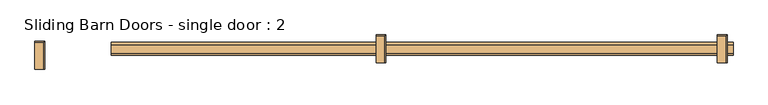
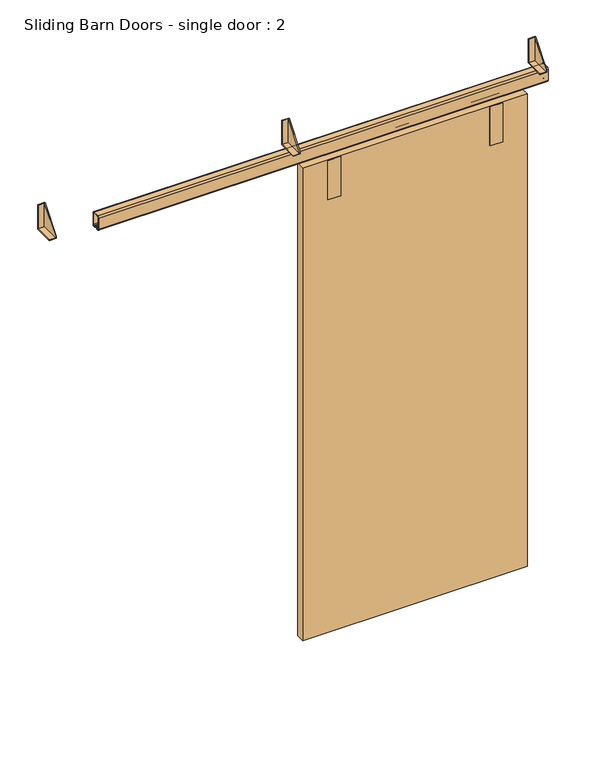
"""IFC4 building model written with IfcOpenShell, lengths in millimetres: door geometry, Sliding Barn Doors - single door : 2."""

from ifc_helpers import new_model, si_unit, point, frame, frame_2d, origin, place, context, project, spatial, polyline, circle_curve, trimmed, segment, composite_curve, outline, extrude, source, transform, mapped, element, save


def sliding_barn_doors_single_door_2_8c843bd4(model_context):
    return source(origin(), model_context, "Body", "SweptSolid", [
        extrude(outline(polyline([(-158.75, 2152.65), (-79.375, 2247.773), (-79.375, 2146.3), (-158.75, 2146.3), (-158.75, 2152.65)])), frame((-1487.5371094, 0.0, 0.0), z_axis=(1.0, 0.0, 0.0), x_axis=(0.0, 1.0, 0.0)), (0.0, 0.0, 1.0), 3.175),
        extrude(outline(polyline([(-76.2, 2143.125), (-158.75, 2143.125), (-158.75, 2146.3), (-79.375, 2146.3), (-79.375, 2247.773), (-76.2, 2247.773), (-76.2, 2143.125)])), frame((-1512.8378906, 0.0, 0.0), z_axis=(1.0, 0.0, 0.0), x_axis=(0.0, 1.0, 0.0)), (0.0, 0.0, 1.0), 28.4757812),
        extrude(outline(polyline([(-139.7, 2152.65), (-60.325, 2247.773), (-60.325, 2146.3), (-139.7, 2146.3), (-139.7, 2152.65)])), frame((-484.2371094, 0.0, 0.0), z_axis=(1.0, 0.0, 0.0), x_axis=(0.0, 1.0, 0.0)), (0.0, 0.0, 1.0), 3.175),
        extrude(outline(polyline([(-57.15, 2143.125), (-139.7, 2143.125), (-139.7, 2146.3), (-60.325, 2146.3), (-60.325, 2247.773), (-57.15, 2247.773), (-57.15, 2143.125)])), frame((-509.5378906, 0.0, 0.0), z_axis=(1.0, 0.0, 0.0), x_axis=(0.0, 1.0, 0.0)), (0.0, 0.0, 1.0), 28.4757813),
        extrude(outline(polyline([(-139.7, 2152.65), (-60.325, 2247.773), (-60.325, 2146.3), (-139.7, 2146.3), (-139.7, 2152.65)])), frame((519.0628906, 0.0, 0.0), z_axis=(1.0, 0.0, 0.0), x_axis=(0.0, 1.0, 0.0)), (0.0, 0.0, 1.0), 3.175),
        extrude(outline(polyline([(-57.15, 2143.125), (-139.7, 2143.125), (-139.7, 2146.3), (-60.325, 2146.3), (-60.325, 2247.773), (-57.15, 2247.773), (-57.15, 2143.125)])), frame((493.7621094, 0.0, 0.0), z_axis=(1.0, 0.0, 0.0), x_axis=(0.0, 1.0, 0.0)), (0.0, 0.0, 1.0), 28.4757813),
        extrude(outline(polyline([(-355.854, -117.475), (-355.854, -114.3), (-304.546, -114.3), (-304.546, -117.475), (-355.854, -117.475)])), frame((0.0, 0.0, 1889.252), z_axis=(0.0, 0.0, 1.0), x_axis=(1.0, 0.0, 0.0)), (0.0, 0.0, 1.0), 168.148),
        extrude(outline(polyline([(304.546, -117.475), (304.546, -114.3), (355.854, -114.3), (355.854, -117.475), (304.546, -117.475)])), frame((0.0, 0.0, 1889.252), z_axis=(0.0, 0.0, 1.0), x_axis=(1.0, 0.0, 0.0)), (0.0, 0.0, 1.0), 168.148),
        extrude(outline(polyline([(-457.2, -114.3), (-457.2, -79.375), (457.2, -79.375), (457.2, -114.3), (-457.2, -114.3)])), frame((0.0, 0.0, 25.4), z_axis=(0.0, 0.0, 1.0), x_axis=(1.0, 0.0, 0.0)), (0.0, 0.0, 1.0), 2032.0),
        extrude(outline(composite_curve([segment(trimmed(circle_curve(frame_2d((-85.725, 2136.775)), 6.35), [point((-85.725, 2143.125))], [point((-79.375, 2136.775))], False, "CARTESIAN"), True, "CONTINUOUS"), segment(polyline([(-79.375, 2136.775), (-79.375, 2088.515)]), True, "CONTINUOUS"), segment(trimmed(circle_curve(frame_2d((-85.725, 2088.515)), 6.35), [point((-79.375, 2088.515))], [point((-85.725, 2082.165))], False, "CARTESIAN"), True, "CONTINUOUS"), segment(polyline([(-85.725, 2082.165), (-91.1336853, 2082.165)]), True, "CONTINUOUS"), segment(trimmed(circle_curve(frame_2d((-91.1336853, 2083.7525)), 1.5875), [point((-91.1336853, 2082.165))], [point((-92.6920184, 2083.4495907))], False, "CARTESIAN"), True, "CONTINUOUS"), segment(polyline([(-92.6920184, 2083.4495907), (-94.1175341, 2090.7832331), (-92.6013971, 2090.7832331), (-91.2154749, 2083.6532812), (-85.725, 2083.6532812)]), True, "CONTINUOUS"), segment(trimmed(circle_curve(frame_2d((-85.725, 2088.515)), 4.8617187), [point((-85.725, 2083.6532812))], [point((-80.8632813, 2088.515))], True, "CARTESIAN"), True, "CONTINUOUS"), segment(polyline([(-80.8632813, 2088.515), (-80.8632813, 2136.775)]), True, "CONTINUOUS"), segment(trimmed(circle_curve(frame_2d((-85.725, 2136.775)), 4.8617187), [point((-80.8632813, 2136.775))], [point((-85.725, 2141.6367187))], True, "CARTESIAN"), True, "CONTINUOUS"), segment(polyline([(-85.725, 2141.6367187), (-111.252, 2141.6367187)]), True, "CONTINUOUS"), segment(trimmed(circle_curve(frame_2d((-111.252, 2136.775)), 4.8617187), [point((-111.252, 2141.6367187))], [point((-116.1137188, 2136.775))], True, "CARTESIAN"), True, "CONTINUOUS"), segment(polyline([(-116.1137188, 2136.775), (-116.1137188, 2088.515)]), True, "CONTINUOUS"), segment(trimmed(circle_curve(frame_2d((-111.252, 2088.515)), 4.8617187), [point((-116.1137188, 2088.515))], [point((-111.252, 2083.6532812))], True, "CARTESIAN"), True, "CONTINUOUS"), segment(polyline([(-111.252, 2083.6532812), (-105.7615251, 2083.6532812), (-104.3756029, 2090.7832331), (-102.8594659, 2090.7832331), (-104.2849816, 2083.4495907)]), True, "CONTINUOUS"), segment(trimmed(circle_curve(frame_2d((-105.8433147, 2083.7525)), 1.5875), [point((-104.2849816, 2083.4495907))], [point((-105.8433147, 2082.165))], False, "CARTESIAN"), True, "CONTINUOUS"), segment(polyline([(-105.8433147, 2082.165), (-111.252, 2082.165)]), True, "CONTINUOUS"), segment(trimmed(circle_curve(frame_2d((-111.252, 2088.515)), 6.35), [point((-111.252, 2082.165))], [point((-117.602, 2088.515))], False, "CARTESIAN"), True, "CONTINUOUS"), segment(polyline([(-117.602, 2088.515), (-117.602, 2136.775)]), True, "CONTINUOUS"), segment(trimmed(circle_curve(frame_2d((-111.252, 2136.775)), 6.35), [point((-117.602, 2136.775))], [point((-111.252, 2143.125))], False, "CARTESIAN"), True, "CONTINUOUS"), segment(polyline([(-111.252, 2143.125), (-85.725, 2143.125)]), True, "CONTINUOUS")], self_intersect=False)), frame((-1289.05, 0.0, 0.0), z_axis=(1.0, 0.0, 0.0), x_axis=(0.0, 1.0, 0.0)), (0.0, 0.0, 1.0), 1828.8),
    ])


if __name__ == "__main__":
    model = new_model("IFC4")
    model_context = context("Model", 3, world=origin())
    ifc_project = project(units=[si_unit("LENGTHUNIT", "METRE", prefix="MILLI")], contexts=[model_context])
    site = spatial("IfcSite", under=ifc_project)
    building = spatial("IfcBuilding", under=site)
    placement = place(None, origin())
    sliding_barn_doors_single_door_2_shape = sliding_barn_doors_single_door_2_8c843bd4(model_context)
    element("IfcDoor", 1, ObjectType="Sliding Barn Doors - single door : 2", at=placement, inside=building, context=model_context, shape_type="MappedRepresentation", body=[
        mapped(sliding_barn_doors_single_door_2_shape, transform((0.0, 0.0, 0.0), x_axis=(1.0, 0.0, 0.0), y_axis=(0.0, 1.0, 0.0), z_axis=(0.0, 0.0, 1.0))),
    ])
    save(model, "model.ifc")

# Revit data of these elements
# Type "Sliding Barn Doors - single door : 2"
#   Type Mark = "62"
#   OD_DS_Door_Material = "T.B.D."
#   OD_DS_Door_Type = "SLIDER"
#   OD_DS_Lockset = "-"
#   Analytic Construction = "<None>"
#   rail_overlap_left = 0' - 5 1/4"
#   rail_length = 6' - 0"
#   overlap_left = 0' - 2"
#   overlap = 0' - 0"
#   bracket_right = 3' - 7"
#   bracket_left = 0' - 4"
#   Thickness = 0' - 1 3/8"
#   Panel Width = 3' - 0"
#   Panel Height = 6' - 8"
#   Gap 2 = 0' - 0 1/2"
#   Gap 1 = 0' - 0 7/8"
#   Frame Projection Ext. = 0' - 1"
#   Frame Projection Int. = 0' - 1"
#   Frame Width = 0' - 3"
#   Height = 6' - 4"
#   Width = 2' - 8"
#   Bracket_offset = 0' - 5"
#   Door_4 = no
#   Door_3 = no
#   Hardware Material = Metal - Aluminum
#   Door Material = Closet_1
#   Function = (empty or 0)
#   Wall Closure = (empty or 0)
# Element 1 (IfcDoor, "Sliding Barn Doors - single door : 2")
#   Materials on its faces: "Metal - Aluminum", "Closet_1"
# Materials
#   "Metal - Aluminum": class "Metal", colour RGB 247 247 247, transparency 0
#   "Closet_1": class "Paint", colour RGB 200 194 183, transparency 0, Cost = 0
